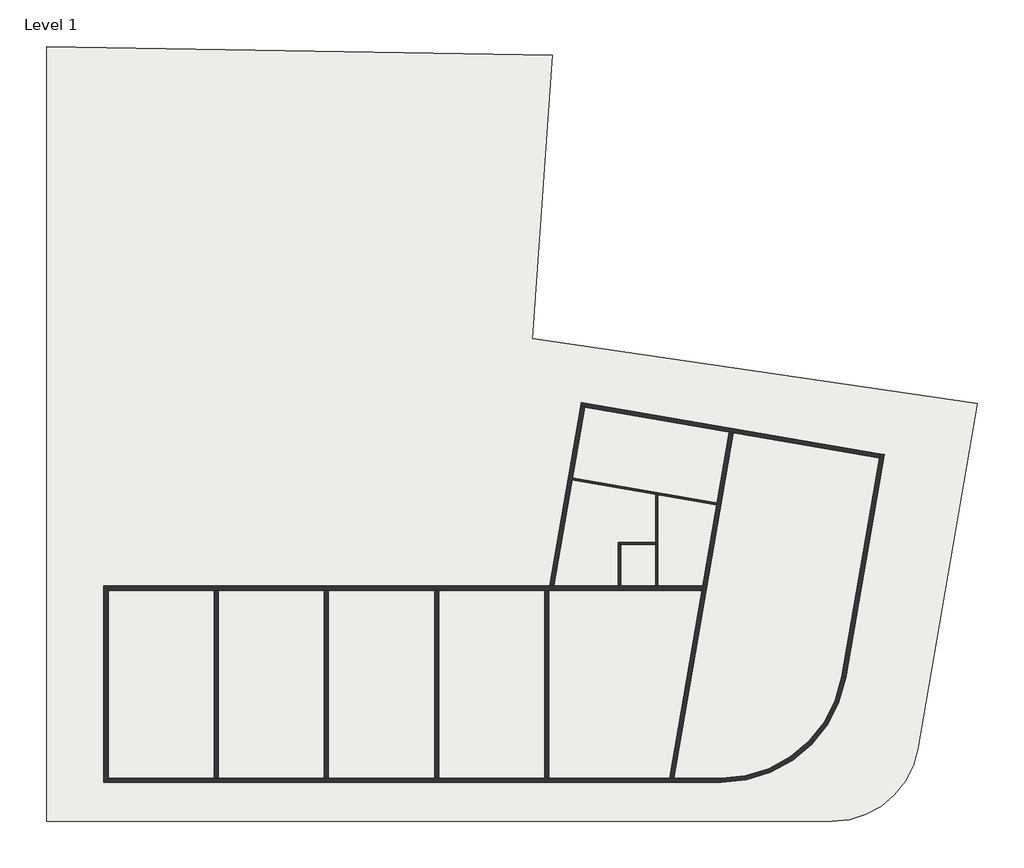
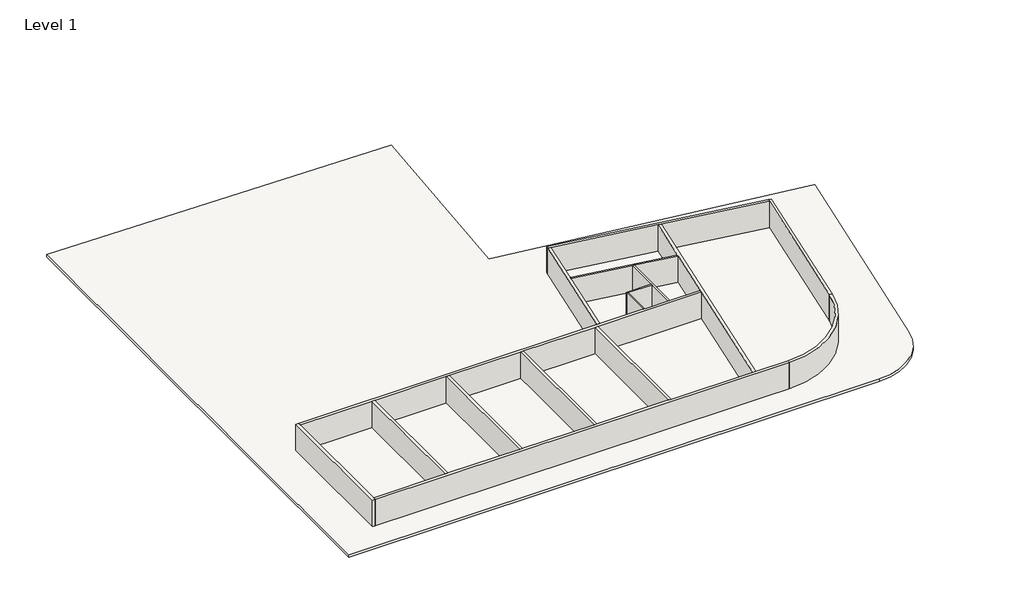
# One storey: 16 walls, 1 slab.
"""IFC4 building model written with IfcOpenShell, lengths in millimetres."""

from ifc_helpers import new_model, si_unit, point, frame, frame_2d, origin, origin_with_axes, place, context, project, spatial, polyline, circle_curve, trimmed, segment, composite_curve, outline, extrude, faceted_brep, element, save

model = new_model("IFC4")

# Units and contexts
model_context = context("Model", 3, world=origin())
ifc_project = project(units=[si_unit("LENGTHUNIT", "METRE", prefix="MILLI")], contexts=[model_context])

# Site, building, storey
site = spatial("IfcSite", under=ifc_project)
building = spatial("IfcBuilding", under=site)
storey = spatial("IfcBuildingStorey", under=building, Name="Level 1", Elevation=0.0)

# Slab
placement = place(None, origin())
element("IfcSlab", 1, ObjectType="Site_Boundary", at=placement, inside=storey, context=model_context, shape_type="SweptSolid", body=[
    extrude(outline(composite_curve([segment(polyline([(34835.2447432, -3925.2102531), (-22915.1714845, -3925.2102531), (-22915.1714845, 53072.3897469), (14264.7649685, 52423.4115421), (12808.3335045, 31595.4712495), (45529.7971898, 26801.3470403), (41142.7609558, 1386.7923054)]), True, "CONTINUOUS"), segment(trimmed(circle_curve(frame_2d((34835.2447432, 2475.5897469)), 6400.8), [point((41142.7609558, 1386.7923054))], [point((34835.2447432, -3925.2102531))], False, "CARTESIAN"), True, "CONTINUOUS")], self_intersect=False)), frame((0.0, 0.0, -304.8), z_axis=(0.0, 0.0, 1.0), x_axis=(1.0, 0.0, 0.0)), (0.0, 0.0, 1.0), 304.8),
])

# Walls
element("IfcWall", 2, ObjectType="Generic - 12\"", at=placement, inside=storey, context=model_context, shape_type="Brep", body=[
    faceted_brep([(-18396.0353714, -1072.2068004, 0.0), (-18396.0353714, -767.4068004, 0.0), (-18396.0353714, 13070.5131996, 0.0), (-18396.0353714, 13375.3131996, 0.0), (-18396.0353714, 13375.3131996, 3048.0), (-18396.0353714, 13070.5131996, 3048.0), (-18396.0353714, -767.4068004, 3048.0), (-18396.0353714, -1072.2068004, 3048.0), (-18700.8353714, -1072.2068004, 0.0), (-18700.8353714, -1072.2068004, 3048.0), (-18700.8353714, 13375.3131996, 3048.0), (-18700.8353714, 13375.3131996, 0.0)], [[[0, 1, 2, 3, 4, 5, 6, 7]], [[8, 9, 10, 11]], [[3, 2, 1, 0, 8, 11]], [[7, 6, 5, 4, 10, 9]], [[4, 3, 11, 10]], [[0, 7, 9, 8]]]),
])
element("IfcWall", 3, ObjectType="Generic - 12\"", at=placement, inside=storey, context=model_context, shape_type="Brep", body=[
    faceted_brep([(-18396.0353714, 13070.5131996, 0.0), (-10597.2193714, 13070.5131996, 0.0), (-10292.4193714, 13070.5131996, 0.0), (-2493.6033714, 13070.5131996, 0.0), (-2188.8033714, 13070.5131996, 0.0), (5610.0126286, 13070.5131996, 0.0), (5914.8126286, 13070.5131996, 0.0), (13713.6286286, 13070.5131996, 0.0), (14018.4286286, 13070.5131996, 0.0), (25281.5464527, 13070.5131996, 0.0), (25281.5464527, 13070.5131996, 3048.0), (14018.4286286, 13070.5131996, 3048.0), (13713.6286286, 13070.5131996, 3048.0), (5914.8126286, 13070.5131996, 3048.0), (5610.0126286, 13070.5131996, 3048.0), (-2188.8033714, 13070.5131996, 3048.0), (-2493.6033714, 13070.5131996, 3048.0), (-10292.4193714, 13070.5131996, 3048.0), (-10597.2193714, 13070.5131996, 3048.0), (-18396.0353714, 13070.5131996, 3048.0), (-18396.0353714, 13375.3131996, 0.0), (-18396.0353714, 13375.3131996, 3048.0), (14082.1915445, 13375.3131996, 3048.0), (14391.499325, 13375.3131996, 3048.0), (19132.7040087, 13375.3131996, 3048.0), (19285.1040087, 13375.3131996, 3048.0), (21875.9040087, 13375.3131996, 3048.0), (22028.3040087, 13375.3131996, 3048.0), (25334.1607384, 13375.3131996, 3048.0), (25334.1607384, 13375.3131996, 0.0), (22028.3040087, 13375.3131996, 0.0), (21875.9040087, 13375.3131996, 0.0), (19285.1040087, 13375.3131996, 0.0), (19132.7040087, 13375.3131996, 0.0), (14391.499325, 13375.3131996, 0.0), (14082.1915445, 13375.3131996, 0.0)], [[[0, 1, 2, 3, 4, 5, 6, 7, 8, 9, 10, 11, 12, 13, 14, 15, 16, 17, 18, 19]], [[20, 21, 22, 23, 24, 25, 26, 27, 28, 29, 30, 31, 32, 33, 34, 35]], [[9, 8, 7, 6, 5, 4, 3, 2, 1, 0, 20, 35, 34, 33, 32, 31, 30, 29]], [[19, 18, 17, 16, 15, 14, 13, 12, 11, 10, 28, 27, 26, 25, 24, 23, 22, 21]], [[0, 19, 21, 20]], [[10, 9, 29, 28]]]),
])
element("IfcWall", 4, ObjectType="Generic - 12\"", at=placement, inside=storey, context=model_context, shape_type="Brep", body=[
    faceted_brep([(-18396.0353714, -1072.2068004, 0.0), (26683.8783962, -1072.2068004, 0.0), (26683.8783962, -1072.2068004, 3048.0), (-18396.0353714, -1072.2068004, 3048.0), (-18396.0353714, -767.4068004, 0.0), (-18396.0353714, -767.4068004, 3048.0), (-10597.2193714, -767.4068004, 3048.0), (-10292.4193714, -767.4068004, 3048.0), (-2493.6033714, -767.4068004, 3048.0), (-2188.8033714, -767.4068004, 3048.0), (5610.0126286, -767.4068004, 3048.0), (5914.8126286, -767.4068004, 3048.0), (13713.6286286, -767.4068004, 3048.0), (14018.4286286, -767.4068004, 3048.0), (22892.8578813, -767.4068004, 3048.0), (23202.1656617, -767.4068004, 3048.0), (26683.8783962, -767.4068004, 3048.0), (26683.8783962, -767.4068004, 0.0), (23202.1656617, -767.4068004, 0.0), (22892.8578813, -767.4068004, 0.0), (14018.4286286, -767.4068004, 0.0), (13713.6286286, -767.4068004, 0.0), (5914.8126286, -767.4068004, 0.0), (5610.0126286, -767.4068004, 0.0), (-2188.8033714, -767.4068004, 0.0), (-2493.6033714, -767.4068004, 0.0), (-10292.4193714, -767.4068004, 0.0), (-10597.2193714, -767.4068004, 0.0)], [[[0, 1, 2, 3]], [[4, 5, 6, 7, 8, 9, 10, 11, 12, 13, 14, 15, 16, 17, 18, 19, 20, 21, 22, 23, 24, 25, 26, 27]], [[1, 0, 4, 27, 26, 25, 24, 23, 22, 21, 20, 19, 18, 17]], [[2, 1, 17, 16]], [[3, 2, 16, 15, 14, 13, 12, 11, 10, 9, 8, 7, 6, 5]], [[0, 3, 5, 4]]]),
])
element("IfcWall", 5, ObjectType="Generic - 12\"", at=placement, inside=storey, context=model_context, shape_type="Brep", body=[
    faceted_brep([(35844.7948001, 6642.8445346, 0.0), (38677.893346, 23055.2774898, 0.0), (38677.893346, 23055.2774898, 3048.0), (35844.7948001, 6642.8445346, 3048.0), (35544.4368852, 6694.6920318, 0.0), (35544.4368852, 6694.6920318, 3048.0), (38325.6879339, 22806.7670721, 3048.0), (38377.5354311, 23107.124987, 3048.0), (38377.5354311, 23107.124987, 0.0), (38325.6879339, 22806.7670721, 0.0)], [[[0, 1, 2, 3]], [[4, 5, 6, 7, 8, 9]], [[1, 0, 4, 9, 8]], [[3, 2, 7, 6, 5]], [[0, 3, 5, 4]], [[2, 1, 8, 7]]]),
])
element("IfcWall", 6, ObjectType="Generic - 12\"", at=placement, inside=storey, context=model_context, shape_type="Brep", body=[
    faceted_brep([(38377.5354311, 23107.124987, 0.0), (16416.4688965, 26898.0233769, 0.0), (16416.4688965, 26898.0233769, 3048.0), (38377.5354311, 23107.124987, 3048.0), (16364.6213993, 26597.665462, 0.0), (16664.9793142, 26545.8179648, 0.0), (27291.013229, 24711.5621105, 0.0), (27591.3711438, 24659.7146132, 0.0), (38325.6879339, 22806.7670721, 0.0), (38325.6879339, 22806.7670721, 3048.0), (27591.3711438, 24659.7146132, 3048.0), (27291.013229, 24711.5621105, 3048.0), (16664.9793142, 26545.8179648, 3048.0), (16364.6213993, 26597.665462, 3048.0)], [[[0, 1, 2, 3]], [[4, 5, 6, 7, 8, 9, 10, 11, 12, 13]], [[1, 0, 8, 7, 6, 5, 4]], [[3, 2, 13, 12, 11, 10, 9]], [[0, 3, 9, 8]], [[2, 1, 4, 13]]]),
])
element("IfcWall", 7, ObjectType="Generic - 12\"", at=placement, inside=storey, context=model_context, shape_type="Brep", body=[
    faceted_brep([(14391.499325, 13375.3131996, 0.0), (15738.162384, 21176.6716102, 0.0), (15764.0861326, 21326.8505677, 0.0), (16664.9793142, 26545.8179648, 0.0), (16664.9793142, 26545.8179648, 3048.0), (15764.0861326, 21326.8505677, 3048.0), (15738.162384, 21176.6716102, 3048.0), (14391.499325, 13375.3131996, 3048.0), (16364.6213993, 26597.665462, 0.0), (14082.1915445, 13375.3131996, 0.0), (14082.1915445, 13375.3131996, 3048.0), (16364.6213993, 26597.665462, 3048.0)], [[[0, 1, 2, 3, 4, 5, 6, 7]], [[8, 9, 10, 11]], [[3, 2, 1, 0, 9, 8]], [[7, 6, 5, 4, 11, 10]], [[0, 7, 10, 9]], [[4, 3, 8, 11]]]),
])
element("IfcWall", 8, ObjectType="Generic - 12\"", at=placement, inside=storey, context=model_context, shape_type="SweptSolid", body=[
    extrude(outline(polyline([(14018.4286286, 13070.5131996), (14018.4286286, -767.4068004), (13713.6286286, -767.4068004), (13713.6286286, 13070.5131996), (14018.4286286, 13070.5131996)])), origin_with_axes(), (0.0, 0.0, 1.0), 3048.0),
])
element("IfcWall", 9, ObjectType="Generic - 12\"", at=placement, inside=storey, context=model_context, shape_type="SweptSolid", body=[
    extrude(outline(polyline([(5914.8126286, 13070.5131996), (5914.8126286, -767.4068004), (5610.0126286, -767.4068004), (5610.0126286, 13070.5131996), (5914.8126286, 13070.5131996)])), origin_with_axes(), (0.0, 0.0, 1.0), 3048.0),
])
element("IfcWall", 10, ObjectType="Generic - 12\"", at=placement, inside=storey, context=model_context, shape_type="SweptSolid", body=[
    extrude(outline(polyline([(-2188.8033714, 13070.5131996), (-2188.8033714, -767.4068004), (-2493.6033714, -767.4068004), (-2493.6033714, 13070.5131996), (-2188.8033714, 13070.5131996)])), origin_with_axes(), (0.0, 0.0, 1.0), 3048.0),
])
element("IfcWall", 11, ObjectType="Generic - 12\"", at=placement, inside=storey, context=model_context, shape_type="SweptSolid", body=[
    extrude(outline(polyline([(-10292.4193714, 13070.5131996), (-10292.4193714, -767.4068004), (-10597.2193714, -767.4068004), (-10597.2193714, 13070.5131996), (-10292.4193714, 13070.5131996)])), origin_with_axes(), (0.0, 0.0, 1.0), 3048.0),
])
element("IfcWall", 12, ObjectType="Generic - 12\"", at=placement, inside=storey, context=model_context, shape_type="Brep", body=[
    faceted_brep([(23202.1656617, -767.4068004, 0.0), (27591.3711438, 24659.7146132, 0.0), (27591.3711438, 24659.7146132, 3048.0), (23202.1656617, -767.4068004, 3048.0), (22892.8578813, -767.4068004, 3048.0), (25281.5464527, 13070.5131996, 3048.0), (25334.1607384, 13375.3131996, 3048.0), (26364.1962987, 19342.4157559, 3048.0), (26390.1200473, 19492.5947134, 3048.0), (27291.013229, 24711.5621105, 3048.0), (27291.013229, 24711.5621105, 0.0), (26390.1200473, 19492.5947134, 0.0), (26364.1962987, 19342.4157559, 0.0), (25334.1607384, 13375.3131996, 0.0), (25281.5464527, 13070.5131996, 0.0), (22892.8578813, -767.4068004, 0.0)], [[[0, 1, 2, 3]], [[4, 5, 6, 7, 8, 9, 10, 11, 12, 13, 14, 15]], [[1, 0, 15, 14, 13, 12, 11, 10]], [[3, 2, 9, 8, 7, 6, 5, 4]], [[0, 3, 4, 15]], [[2, 1, 10, 9]]]),
])
element("IfcWall", 13, ObjectType="Generic - 12\"", at=placement, inside=storey, context=model_context, shape_type="SweptSolid", body=[
    extrude(outline(composite_curve([segment(polyline([(35544.4368852, 6694.6920318), (35844.7948001, 6642.8445346)]), True, "CONTINUOUS"), segment(trimmed(circle_curve(frame_2d((26683.8783962, 8224.1931996)), 9296.4), [point((35844.7948001, 6642.8445346))], [point((26683.8783962, -1072.2068004))], False, "CARTESIAN"), True, "CONTINUOUS"), segment(polyline([(26683.8783962, -1072.2068004), (26683.8783962, -767.4068004)]), True, "CONTINUOUS"), segment(trimmed(circle_curve(frame_2d((26683.8783962, 8224.1931996)), 8991.6), [point((26683.8783962, -767.4068004))], [point((35544.4368852, 6694.6920318))], True, "CARTESIAN"), True, "CONTINUOUS")], self_intersect=False)), origin_with_axes(), (0.0, 0.0, 1.0), 3048.0),
])
element("IfcWall", 14, ObjectType="Generic - 6\"", at=placement, inside=storey, context=model_context, shape_type="Brep", body=[
    faceted_brep([(15738.162384, 21176.6716102, 0.0), (21875.9040087, 20117.1804965, 0.0), (22028.3040087, 20090.8733536, 0.0), (26364.1962987, 19342.4157559, 0.0), (26364.1962987, 19342.4157559, 3048.0), (22028.3040087, 20090.8733536, 3048.0), (21875.9040087, 20117.1804965, 3048.0), (15738.162384, 21176.6716102, 3048.0), (15764.0861326, 21326.8505677, 0.0), (15764.0861326, 21326.8505677, 3048.0), (26390.1200473, 19492.5947134, 3048.0), (26390.1200473, 19492.5947134, 0.0)], [[[0, 1, 2, 3, 4, 5, 6, 7]], [[8, 9, 10, 11]], [[3, 2, 1, 0, 8, 11]], [[7, 6, 5, 4, 10, 9]], [[0, 7, 9, 8]], [[4, 3, 11, 10]]]),
])
element("IfcWall", 15, ObjectType="Generic - 6\"", at=placement, inside=storey, context=model_context, shape_type="Brep", body=[
    faceted_brep([(21875.9040087, 20117.1804965, 0.0), (21875.9040087, 16586.8837362, 0.0), (21875.9040087, 16434.4837362, 0.0), (21875.9040087, 13375.3131996, 0.0), (21875.9040087, 13375.3131996, 3048.0), (21875.9040087, 16434.4837362, 3048.0), (21875.9040087, 16586.8837362, 3048.0), (21875.9040087, 20117.1804965, 3048.0), (22028.3040087, 20090.8733536, 0.0), (22028.3040087, 20090.8733536, 3048.0), (22028.3040087, 13375.3131996, 3048.0), (22028.3040087, 13375.3131996, 0.0)], [[[0, 1, 2, 3, 4, 5, 6, 7]], [[8, 9, 10, 11]], [[3, 2, 1, 0, 8, 11]], [[7, 6, 5, 4, 10, 9]], [[4, 3, 11, 10]], [[0, 7, 9, 8]]]),
])
element("IfcWall", 16, ObjectType="Generic - 6\"", at=placement, inside=storey, context=model_context, shape_type="Brep", body=[
    faceted_brep([(21875.9040087, 16586.8837362, 0.0), (19132.7040087, 16586.8837362, 0.0), (19132.7040087, 16586.8837362, 3048.0), (21875.9040087, 16586.8837362, 3048.0), (21875.9040087, 16434.4837362, 0.0), (21875.9040087, 16434.4837362, 3048.0), (19285.1040087, 16434.4837362, 3048.0), (19132.7040087, 16434.4837362, 3048.0), (19132.7040087, 16434.4837362, 0.0), (19285.1040087, 16434.4837362, 0.0)], [[[0, 1, 2, 3]], [[4, 5, 6, 7, 8, 9]], [[1, 0, 4, 9, 8]], [[3, 2, 7, 6, 5]], [[0, 3, 5, 4]], [[2, 1, 8, 7]]]),
])
element("IfcWall", 17, ObjectType="Generic - 6\"", at=placement, inside=storey, context=model_context, shape_type="SweptSolid", body=[
    extrude(outline(polyline([(19132.7040087, 13375.3131996), (19132.7040087, 16434.4837362), (19285.1040087, 16434.4837362), (19285.1040087, 13375.3131996), (19132.7040087, 13375.3131996)])), origin_with_axes(), (0.0, 0.0, 1.0), 3048.0),
])

save(model, "model.ifc")

# Revit data of these elements
# Project information
#   Project Issue Date = "Issue Date"
#   Project Status = "Project Status"
#   Client Name = "Owner"
#   Project Address = "Enter address here"
#   Project Name = "Project Name"
#   Project Number = "Project Number"
# Grids (mm)
#   "C": line (14938.226, 26998.542) -> (46114.303, 21616.958)
#   "1": line (-18548.435, 18831.233) -> (-18548.435, -7137.727)
#   "2": line (-10444.819, 18831.233) -> (-10444.819, -7137.727)
#   "3": line (-2341.203, 18831.233) -> (-2341.203, -7137.727)
#   "4": line (5762.413, 18831.233) -> (5762.413, -7137.727)
#   "5": line (13866.029, 15344.617) -> (13866.029, -7137.727)
#   "6": line (28835.29, 32761.793) -> (21947.873, -7137.727)
#   "7": line (39869.965, 30856.998) -> (33311.352, -7137.727)
#   "8": line (17908.899, 34647.897) -> (14200.57, 13165.165)
#   "A": line (42224.028, -919.807) -> (-21791.507, -919.807)
#   "B": line (44665.331, 13222.913) -> (-21791.507, 13222.913)
# Type "Site_Boundary"
#   Assembly Code = "B1010"
#   Function = 1
#   Layers, outside or top first: 1' - 0" "Site Boundary" (function 1)
# Type "Generic - 12\""
#   Assembly Code = "B2010"
#   Layers, outside or top first: 1' - 0" no material (function 1)
# Type "Generic - 6\""
#   Assembly Code = "B2010"
#   Layers, outside or top first: 0' - 6" no material (function 1)
# Element 1 (IfcSlab, "Site_Boundary")
#   Height Offset From Level = 0' - 0"
#   Phase Created = New Construction
#   Materials on its faces: "Site Boundary"
# Elements 2, 3, 4, 5, 6, 7, 8, 9, 10, 11, 12 (IfcWall, "Generic - 12\"")
#   Top Offset = 0' - 0"
#   Base Offset = 0' - 0"
#   wall height = 10' - 0"
#   Phase Created = New Construction
#   Base Constraint = Level 1
#   Top Constraint = Level 2
#   Materials on its faces: "Default Wall"
# Element 13 (IfcWall, "Generic - 12\"")
#   Top Offset = 0' - 0"
#   Base Offset = 0' - 0"
#   Unconnected Height = 20' - 0"
#   wall height = 10' - 0"
#   Phase Created = New Construction
#   Materials on its faces: "Default Wall"
# Elements 14, 15, 16, 17 (IfcWall, "Generic - 6\"")
#   Top Offset = 0' - 0"
#   Base Offset = 0' - 0"
#   wall height = 10' - 0"
#   Phase Created = New Construction
#   Base Constraint = Level 1
#   Top Constraint = Level 2
#   Materials on its faces: "Default Wall"
# Materials
#   "Site Boundary": class "Paint", colour RGB 195 52 38, transparency 0, Description = "Steel, paint finish, red, glossy", Cost = 0
#   "Default Wall": class "Miscellaneous", colour RGB 128 128 128, transparency 0, Cost = 0
